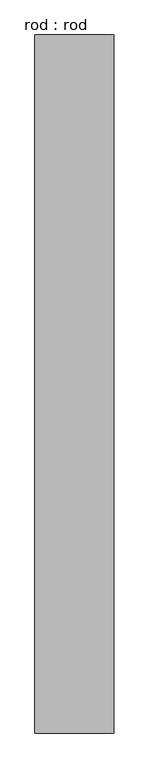
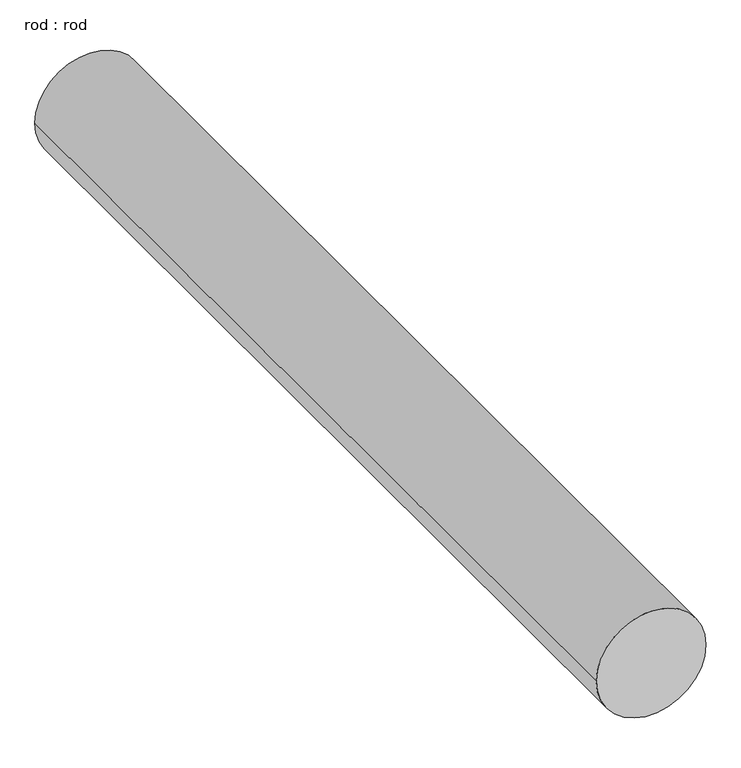
"""IFC4 building model written with IfcOpenShell, lengths in millimetres: proxy geometry, rod : rod."""

from ifc_helpers import new_model, si_unit, point, frame, frame_2d, origin, place, context, project, spatial, circle_curve, trimmed, segment, composite_curve, outline, extrude, source, transform, mapped, element, save


def rod_rod_addac542(model_context):
    return source(origin(), model_context, "Body", "SweptSolid", [
        extrude(outline(composite_curve([segment(trimmed(circle_curve(frame_2d((0.0108462, 0.0)), 200.0), [point((0.0108462, 200.0))], [point((0.0108462, -200.0))], False, "CARTESIAN"), True, "CONTINUOUS"), segment(trimmed(circle_curve(frame_2d((0.0108462, 0.0)), 200.0), [point((0.0108462, -200.0))], [point((0.0108462, 200.0))], False, "CARTESIAN"), True, "CONTINUOUS")], self_intersect=False)), frame((0.0, 2319.5143296, 0.0), z_axis=(0.0, 1.0, 0.0), x_axis=(0.0, 0.0, 1.0)), (0.0, 0.0, 1.0), 3546.4285714),
    ])


if __name__ == "__main__":
    model = new_model("IFC4")
    model_context = context("Model", 3, world=origin())
    ifc_project = project(units=[si_unit("LENGTHUNIT", "METRE", prefix="MILLI")], contexts=[model_context])
    site = spatial("IfcSite", under=ifc_project)
    building = spatial("IfcBuilding", under=site)
    placement = place(None, origin())
    rod_rod_shape = rod_rod_addac542(model_context)
    element("IfcBuildingElementProxy", 1, Name="rod : rod", ObjectType="rod : rod", at=placement, inside=building, context=model_context, shape_type="MappedRepresentation", body=[
        mapped(rod_rod_shape, transform((0.0, 0.0, 0.0), x_axis=(1.0, 0.0, 0.0), y_axis=(0.0, 1.0, 0.0), z_axis=(0.0, 0.0, 1.0))),
    ])
    save(model, "model.ifc")

# Revit data of these elements
# Type "rod : rod"
#   Default Elevation = 0
